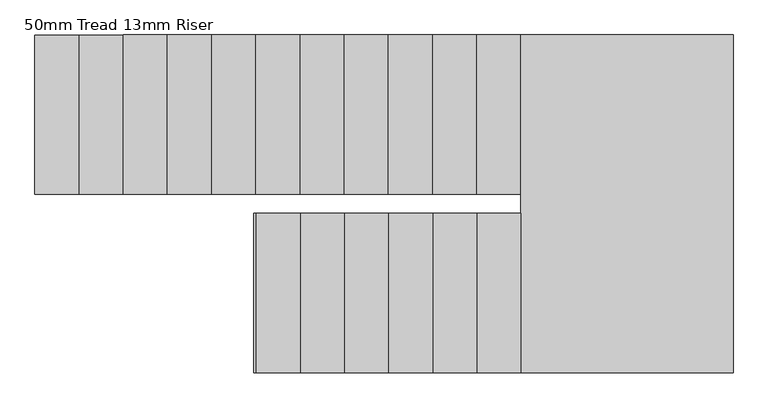
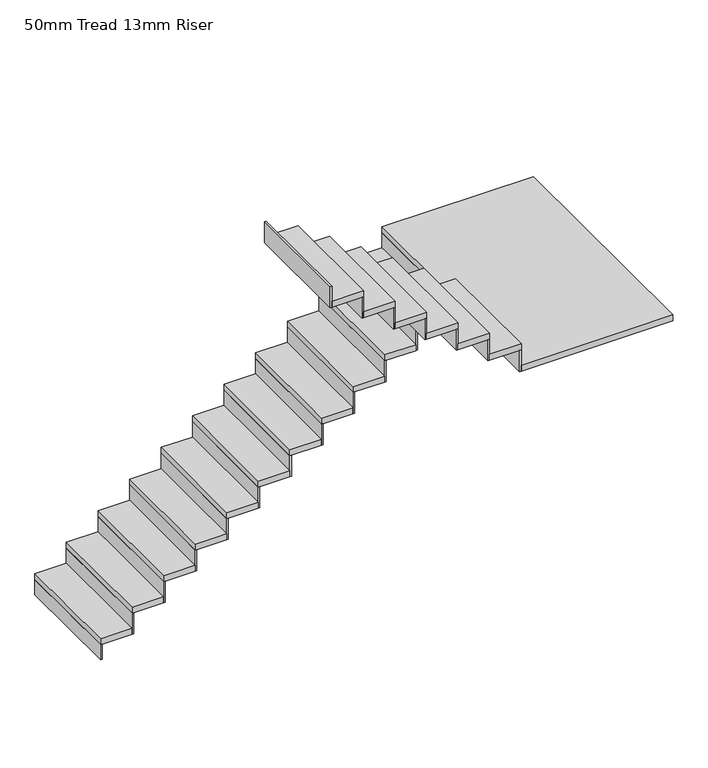
"""IFC4 building model written with IfcOpenShell, lengths in millimetres: stair flight geometry, 50mm Tread 13mm Riser."""

from ifc_helpers import new_model, si_unit, frame, origin, place, context, project, spatial, polyline, outline, extrude, source, transform, mapped, element, save


def stair_flight_50mm_tread_13mm_riser_300e85a3(model_context):
    return source(origin(), model_context, "Body", "SweptSolid", [
        extrude(outline(polyline([(-12784.0903863, 2815.0066114), (-12796.5903863, 2815.0066114), (-12796.5903863, 3715.0066114), (-12784.0903863, 3715.0066114), (-12784.0903863, 2815.0066114)])), frame((0.0, 0.0, 450.0), z_axis=(0.0, 0.0, 1.0), x_axis=(1.0, 0.0, 0.0)), (0.0, 0.0, 1.0), 126.4705882),
        extrude(outline(polyline([(-12546.5903863, 3715.0066114), (-12546.5903863, 2815.0066114), (-12796.5903863, 2815.0066114), (-12796.5903863, 3715.0066114), (-12546.5903863, 3715.0066114)])), frame((0.0, 0.0, 576.4705882), z_axis=(0.0, 0.0, 1.0), x_axis=(1.0, 0.0, 0.0)), (0.0, 0.0, 1.0), 50.0),
        extrude(outline(polyline([(-12534.0903863, 2815.0066114), (-12546.5903863, 2815.0066114), (-12546.5903863, 3715.0066114), (-12534.0903863, 3715.0066114), (-12534.0903863, 2815.0066114)])), frame((0.0, 0.0, 576.4705882), z_axis=(0.0, 0.0, 1.0), x_axis=(1.0, 0.0, 0.0)), (0.0, 0.0, 1.0), 176.4705882),
        extrude(outline(polyline([(-12296.5903863, 3715.0066114), (-12296.5903863, 2815.0066114), (-12546.5903863, 2815.0066114), (-12546.5903863, 3715.0066114), (-12296.5903863, 3715.0066114)])), frame((0.0, 0.0, 752.9411765), z_axis=(0.0, 0.0, 1.0), x_axis=(1.0, 0.0, 0.0)), (0.0, 0.0, 1.0), 50.0),
        extrude(outline(polyline([(-12284.0903863, 2815.0066114), (-12296.5903863, 2815.0066114), (-12296.5903863, 3715.0066114), (-12284.0903863, 3715.0066114), (-12284.0903863, 2815.0066114)])), frame((0.0, 0.0, 752.9411765), z_axis=(0.0, 0.0, 1.0), x_axis=(1.0, 0.0, 0.0)), (0.0, 0.0, 1.0), 176.4705882),
        extrude(outline(polyline([(-12046.5903863, 3715.0066114), (-12046.5903863, 2815.0066114), (-12296.5903863, 2815.0066114), (-12296.5903863, 3715.0066114), (-12046.5903863, 3715.0066114)])), frame((0.0, 0.0, 929.4117647), z_axis=(0.0, 0.0, 1.0), x_axis=(1.0, 0.0, 0.0)), (0.0, 0.0, 1.0), 50.0),
        extrude(outline(polyline([(-12034.0903863, 2815.0066114), (-12046.5903863, 2815.0066114), (-12046.5903863, 3715.0066114), (-12034.0903863, 3715.0066114), (-12034.0903863, 2815.0066114)])), frame((0.0, 0.0, 929.4117647), z_axis=(0.0, 0.0, 1.0), x_axis=(1.0, 0.0, 0.0)), (0.0, 0.0, 1.0), 176.4705882),
        extrude(outline(polyline([(-11796.5903863, 3715.0066114), (-11796.5903863, 2815.0066114), (-12046.5903863, 2815.0066114), (-12046.5903863, 3715.0066114), (-11796.5903863, 3715.0066114)])), frame((0.0, 0.0, 1105.8823529), z_axis=(0.0, 0.0, 1.0), x_axis=(1.0, 0.0, 0.0)), (0.0, 0.0, 1.0), 50.0),
        extrude(outline(polyline([(-11784.0903863, 2815.0066114), (-11796.5903863, 2815.0066114), (-11796.5903863, 3715.0066114), (-11784.0903863, 3715.0066114), (-11784.0903863, 2815.0066114)])), frame((0.0, 0.0, 1105.8823529), z_axis=(0.0, 0.0, 1.0), x_axis=(1.0, 0.0, 0.0)), (0.0, 0.0, 1.0), 176.4705882),
        extrude(outline(polyline([(-11546.5903863, 3715.0066114), (-11546.5903863, 2815.0066114), (-11796.5903863, 2815.0066114), (-11796.5903863, 3715.0066114), (-11546.5903863, 3715.0066114)])), frame((0.0, 0.0, 1282.3529412), z_axis=(0.0, 0.0, 1.0), x_axis=(1.0, 0.0, 0.0)), (0.0, 0.0, 1.0), 50.0),
        extrude(outline(polyline([(-11534.0903863, 2815.0066114), (-11546.5903863, 2815.0066114), (-11546.5903863, 3715.0066114), (-11534.0903863, 3715.0066114), (-11534.0903863, 2815.0066114)])), frame((0.0, 0.0, 1282.3529412), z_axis=(0.0, 0.0, 1.0), x_axis=(1.0, 0.0, 0.0)), (0.0, 0.0, 1.0), 176.4705882),
        extrude(outline(polyline([(-11296.5903863, 3715.0066114), (-11296.5903863, 2815.0066114), (-11546.5903863, 2815.0066114), (-11546.5903863, 3715.0066114), (-11296.5903863, 3715.0066114)])), frame((0.0, 0.0, 1458.8235294), z_axis=(0.0, 0.0, 1.0), x_axis=(1.0, 0.0, 0.0)), (0.0, 0.0, 1.0), 50.0),
        extrude(outline(polyline([(-11284.0903863, 2815.0066114), (-11296.5903863, 2815.0066114), (-11296.5903863, 3715.0066114), (-11284.0903863, 3715.0066114), (-11284.0903863, 2815.0066114)])), frame((0.0, 0.0, 1458.8235294), z_axis=(0.0, 0.0, 1.0), x_axis=(1.0, 0.0, 0.0)), (0.0, 0.0, 1.0), 176.4705882),
        extrude(outline(polyline([(-11046.5903863, 3715.0066114), (-11046.5903863, 2815.0066114), (-11296.5903863, 2815.0066114), (-11296.5903863, 3715.0066114), (-11046.5903863, 3715.0066114)])), frame((0.0, 0.0, 1635.2941176), z_axis=(0.0, 0.0, 1.0), x_axis=(1.0, 0.0, 0.0)), (0.0, 0.0, 1.0), 50.0),
        extrude(outline(polyline([(-11034.0903863, 2815.0066114), (-11046.5903863, 2815.0066114), (-11046.5903863, 3715.0066114), (-11034.0903863, 3715.0066114), (-11034.0903863, 2815.0066114)])), frame((0.0, 0.0, 1635.2941176), z_axis=(0.0, 0.0, 1.0), x_axis=(1.0, 0.0, 0.0)), (0.0, 0.0, 1.0), 176.4705882),
        extrude(outline(polyline([(-10796.5903863, 3715.0066114), (-10796.5903863, 2815.0066114), (-11046.5903863, 2815.0066114), (-11046.5903863, 3715.0066114), (-10796.5903863, 3715.0066114)])), frame((0.0, 0.0, 1811.7647059), z_axis=(0.0, 0.0, 1.0), x_axis=(1.0, 0.0, 0.0)), (0.0, 0.0, 1.0), 50.0),
        extrude(outline(polyline([(-10784.0903863, 2815.0066114), (-10796.5903863, 2815.0066114), (-10796.5903863, 3715.0066114), (-10784.0903863, 3715.0066114), (-10784.0903863, 2815.0066114)])), frame((0.0, 0.0, 1811.7647059), z_axis=(0.0, 0.0, 1.0), x_axis=(1.0, 0.0, 0.0)), (0.0, 0.0, 1.0), 176.4705882),
        extrude(outline(polyline([(-10546.5903863, 3715.0066114), (-10546.5903863, 2815.0066114), (-10796.5903863, 2815.0066114), (-10796.5903863, 3715.0066114), (-10546.5903863, 3715.0066114)])), frame((0.0, 0.0, 1988.2352941), z_axis=(0.0, 0.0, 1.0), x_axis=(1.0, 0.0, 0.0)), (0.0, 0.0, 1.0), 50.0),
        extrude(outline(polyline([(-10534.0903863, 2815.0066114), (-10546.5903863, 2815.0066114), (-10546.5903863, 3715.0066114), (-10534.0903863, 3715.0066114), (-10534.0903863, 2815.0066114)])), frame((0.0, 0.0, 1988.2352941), z_axis=(0.0, 0.0, 1.0), x_axis=(1.0, 0.0, 0.0)), (0.0, 0.0, 1.0), 176.4705882),
        extrude(outline(polyline([(-10296.5903863, 3715.0066114), (-10296.5903863, 2815.0066114), (-10546.5903863, 2815.0066114), (-10546.5903863, 3715.0066114), (-10296.5903863, 3715.0066114)])), frame((0.0, 0.0, 2164.7058824), z_axis=(0.0, 0.0, 1.0), x_axis=(1.0, 0.0, 0.0)), (0.0, 0.0, 1.0), 50.0),
        extrude(outline(polyline([(-10284.0903863, 2815.0066114), (-10296.5903863, 2815.0066114), (-10296.5903863, 3715.0066114), (-10284.0903863, 3715.0066114), (-10284.0903863, 2815.0066114)])), frame((0.0, 0.0, 2164.7058824), z_axis=(0.0, 0.0, 1.0), x_axis=(1.0, 0.0, 0.0)), (0.0, 0.0, 1.0), 176.4705882),
        extrude(outline(polyline([(-10046.5903863, 3715.0066114), (-10046.5903863, 2815.0066114), (-10296.5903863, 2815.0066114), (-10296.5903863, 3715.0066114), (-10046.5903863, 3715.0066114)])), frame((0.0, 0.0, 2341.1764706), z_axis=(0.0, 0.0, 1.0), x_axis=(1.0, 0.0, 0.0)), (0.0, 0.0, 1.0), 50.0),
        extrude(outline(polyline([(-10034.0903863, 2815.0066114), (-10046.5903863, 2815.0066114), (-10046.5903863, 3715.0066114), (-10034.0903863, 3715.0066114), (-10034.0903863, 2815.0066114)])), frame((0.0, 0.0, 2341.1764706), z_axis=(0.0, 0.0, 1.0), x_axis=(1.0, 0.0, 0.0)), (0.0, 0.0, 1.0), 176.4705882),
        extrude(outline(polyline([(-10046.5903863, 1805.0066114), (-10046.5903863, 2705.0066114), (-10046.5903863, 2815.0066114), (-10046.5903863, 3715.0066114), (-8846.5903863, 3715.0066114), (-8846.5903863, 1805.0066114), (-10046.5903863, 1805.0066114)])), frame((0.0, 0.0, 2517.6470588), z_axis=(0.0, 0.0, 1.0), x_axis=(1.0, 0.0, 0.0)), (0.0, 0.0, 1.0), 50.0),
        extrude(outline(polyline([(-10059.0903863, 2705.0066114), (-10046.5903863, 2705.0066114), (-10046.5903863, 1805.0066114), (-10059.0903863, 1805.0066114), (-10059.0903863, 2705.0066114)])), frame((0.0, 0.0, 2517.6470588), z_axis=(0.0, 0.0, 1.0), x_axis=(1.0, 0.0, 0.0)), (0.0, 0.0, 1.0), 176.4705882),
        extrude(outline(polyline([(-10296.5903863, 1805.0066114), (-10296.5903863, 2705.0066114), (-10046.5903863, 2705.0066114), (-10046.5903863, 1805.0066114), (-10296.5903863, 1805.0066114)])), frame((0.0, 0.0, 2694.1176471), z_axis=(0.0, 0.0, 1.0), x_axis=(1.0, 0.0, 0.0)), (0.0, 0.0, 1.0), 50.0),
        extrude(outline(polyline([(-10309.0903863, 2705.0066114), (-10296.5903863, 2705.0066114), (-10296.5903863, 1805.0066114), (-10309.0903863, 1805.0066114), (-10309.0903863, 2705.0066114)])), frame((0.0, 0.0, 2694.1176471), z_axis=(0.0, 0.0, 1.0), x_axis=(1.0, 0.0, 0.0)), (0.0, 0.0, 1.0), 176.4705882),
        extrude(outline(polyline([(-10546.5903863, 1805.0066114), (-10546.5903863, 2705.0066114), (-10296.5903863, 2705.0066114), (-10296.5903863, 1805.0066114), (-10546.5903863, 1805.0066114)])), frame((0.0, 0.0, 2870.5882353), z_axis=(0.0, 0.0, 1.0), x_axis=(1.0, 0.0, 0.0)), (0.0, 0.0, 1.0), 50.0),
        extrude(outline(polyline([(-10559.0903863, 2705.0066114), (-10546.5903863, 2705.0066114), (-10546.5903863, 1805.0066114), (-10559.0903863, 1805.0066114), (-10559.0903863, 2705.0066114)])), frame((0.0, 0.0, 2870.5882353), z_axis=(0.0, 0.0, 1.0), x_axis=(1.0, 0.0, 0.0)), (0.0, 0.0, 1.0), 176.4705882),
        extrude(outline(polyline([(-10796.5903863, 1805.0066114), (-10796.5903863, 2705.0066114), (-10546.5903863, 2705.0066114), (-10546.5903863, 1805.0066114), (-10796.5903863, 1805.0066114)])), frame((0.0, 0.0, 3047.0588235), z_axis=(0.0, 0.0, 1.0), x_axis=(1.0, 0.0, 0.0)), (0.0, 0.0, 1.0), 50.0),
        extrude(outline(polyline([(-10809.0903863, 2705.0066114), (-10796.5903863, 2705.0066114), (-10796.5903863, 1805.0066114), (-10809.0903863, 1805.0066114), (-10809.0903863, 2705.0066114)])), frame((0.0, 0.0, 3047.0588235), z_axis=(0.0, 0.0, 1.0), x_axis=(1.0, 0.0, 0.0)), (0.0, 0.0, 1.0), 176.4705882),
        extrude(outline(polyline([(-11046.5903863, 1805.0066114), (-11046.5903863, 2705.0066114), (-10796.5903863, 2705.0066114), (-10796.5903863, 1805.0066114), (-11046.5903863, 1805.0066114)])), frame((0.0, 0.0, 3223.5294118), z_axis=(0.0, 0.0, 1.0), x_axis=(1.0, 0.0, 0.0)), (0.0, 0.0, 1.0), 50.0),
        extrude(outline(polyline([(-11059.0903863, 2705.0066114), (-11046.5903863, 2705.0066114), (-11046.5903863, 1805.0066114), (-11059.0903863, 1805.0066114), (-11059.0903863, 2705.0066114)])), frame((0.0, 0.0, 3223.5294118), z_axis=(0.0, 0.0, 1.0), x_axis=(1.0, 0.0, 0.0)), (0.0, 0.0, 1.0), 176.4705882),
        extrude(outline(polyline([(-11296.5903863, 1805.0066114), (-11296.5903863, 2705.0066114), (-11046.5903863, 2705.0066114), (-11046.5903863, 1805.0066114), (-11296.5903863, 1805.0066114)])), frame((0.0, 0.0, 3400.0), z_axis=(0.0, 0.0, 1.0), x_axis=(1.0, 0.0, 0.0)), (0.0, 0.0, 1.0), 50.0),
        extrude(outline(polyline([(-11309.0903863, 2705.0066114), (-11296.5903863, 2705.0066114), (-11296.5903863, 1805.0066114), (-11309.0903863, 1805.0066114), (-11309.0903863, 2705.0066114)])), frame((0.0, 0.0, 3400.0), z_axis=(0.0, 0.0, 1.0), x_axis=(1.0, 0.0, 0.0)), (0.0, 0.0, 1.0), 176.4705882),
        extrude(outline(polyline([(-11559.0903863, 2705.0066114), (-11546.5903863, 2705.0066114), (-11546.5903863, 1805.0066114), (-11559.0903863, 1805.0066114), (-11559.0903863, 2705.0066114)])), frame((0.0, 0.0, 3576.4705882), z_axis=(0.0, 0.0, 1.0), x_axis=(1.0, 0.0, 0.0)), (0.0, 0.0, 1.0), 176.4705882),
        extrude(outline(polyline([(-11546.5903863, 1805.0066114), (-11546.5903863, 2705.0066114), (-11296.5903863, 2705.0066114), (-11296.5903863, 1805.0066114), (-11546.5903863, 1805.0066114)])), frame((0.0, 0.0, 3576.4705882), z_axis=(0.0, 0.0, 1.0), x_axis=(1.0, 0.0, 0.0)), (0.0, 0.0, 1.0), 50.0),
    ])


if __name__ == "__main__":
    model = new_model("IFC4")
    model_context = context("Model", 3, world=origin())
    ifc_project = project(units=[si_unit("LENGTHUNIT", "METRE", prefix="MILLI")], contexts=[model_context])
    site = spatial("IfcSite", under=ifc_project)
    building = spatial("IfcBuilding", under=site)
    placement = place(None, origin())
    stair_flight_50mm_tread_13mm_riser_shape = stair_flight_50mm_tread_13mm_riser_300e85a3(model_context)
    element("IfcStairFlight", 1, ObjectType="50mm Tread 13mm Riser", at=placement, inside=building, context=model_context, shape_type="MappedRepresentation", body=[
        mapped(stair_flight_50mm_tread_13mm_riser_shape, transform((0.0, 0.0, 0.0), x_axis=(1.0, 0.0, 0.0), y_axis=(0.0, 1.0, 0.0), z_axis=(0.0, 0.0, 1.0))),
    ])
    save(model, "model.ifc")
